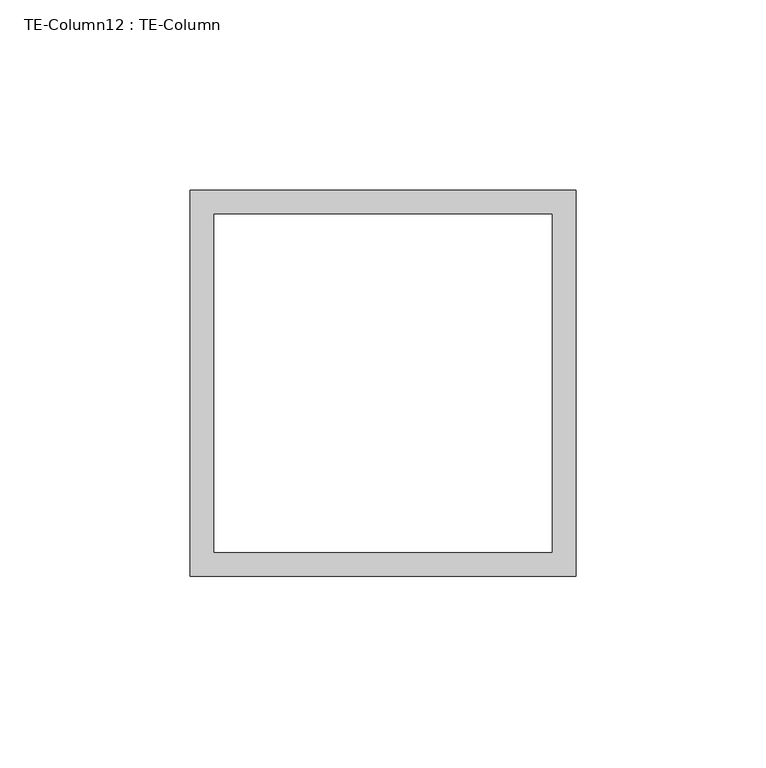
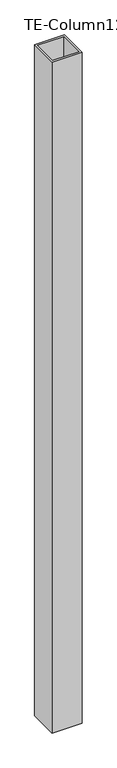
"""IFC4 building model written with IfcOpenShell, lengths in millimetres: proxy geometry, TE-Column12 : TE-Column."""

from ifc_helpers import new_model, si_unit, frame, origin, place, context, project, spatial, polyline, outline, extrude, source, transform, mapped, element, save


def te_column12_te_column_b03e1283(model_context):
    return source(origin(), model_context, "Body", "SweptSolid", [
        extrude(outline(polyline([(590318.6434739, -531667.7913841), (590318.6434739, -531769.3913841), (590217.0434739, -531769.3913841), (590217.0434739, -531667.7913841), (590318.6434739, -531667.7913841)]), holes=[polyline([(590223.3934739, -531674.1413841), (590223.3934739, -531763.0413841), (590312.2934739, -531763.0413841), (590312.2934739, -531674.1413841), (590223.3934739, -531674.1413841)])]), frame((0.0, 0.0, 28.575), z_axis=(0.0, 0.0, 1.0), x_axis=(1.0, 0.0, 0.0)), (0.0, 0.0, 1.0), 2406.65),
    ])


if __name__ == "__main__":
    model = new_model("IFC4")
    model_context = context("Model", 3, world=origin())
    ifc_project = project(units=[si_unit("LENGTHUNIT", "METRE", prefix="MILLI")], contexts=[model_context])
    site = spatial("IfcSite", under=ifc_project)
    building = spatial("IfcBuilding", under=site)
    placement = place(None, origin())
    te_column12_te_column_shape = te_column12_te_column_b03e1283(model_context)
    element("IfcBuildingElementProxy", 1, Name="TE-Column12 : TE-Column", ObjectType="TE-Column12 : TE-Column", at=placement, inside=building, context=model_context, shape_type="MappedRepresentation", body=[
        mapped(te_column12_te_column_shape, transform((0.0, 0.0, 0.0), x_axis=(1.0, 0.0, 0.0), y_axis=(0.0, 1.0, 0.0), z_axis=(0.0, 0.0, 1.0))),
    ])
    save(model, "model.ifc")

# Revit data of these elements
# Element 1 (IfcBuildingElementProxy, "TE-Column12 : TE-Column")
#   Materials on its faces: "4\"X4\" GALV. HSS TUBING"
# Materials
#   "4\"X4\" GALV. HSS TUBING": class "Generic", colour RGB 211 211 207, transparency 0, Cost = 0
